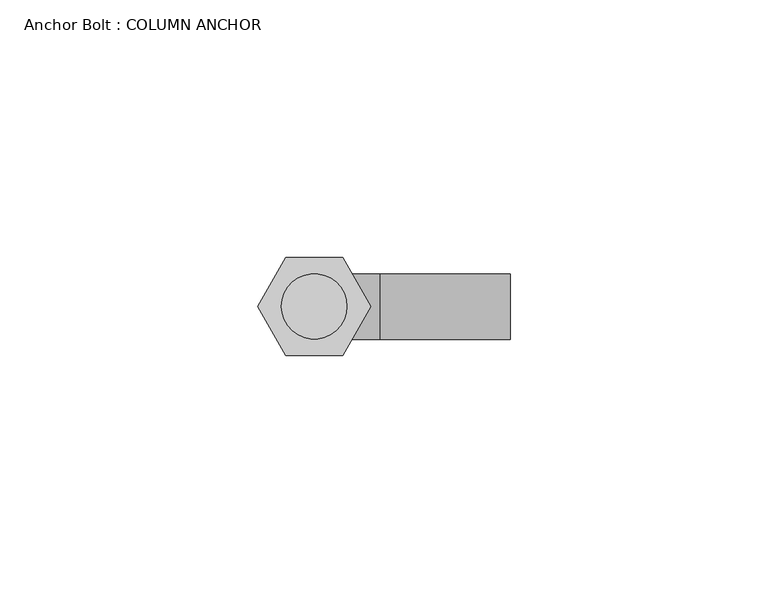
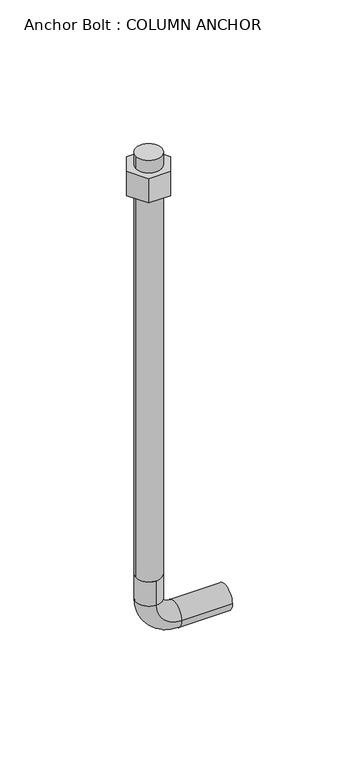
"""IFC4 building model written with IfcOpenShell, lengths in millimetres: fastener geometry, Anchor Bolt : COLUMN ANCHOR."""

from ifc_helpers import new_model, si_unit, point, frame, origin, origin_with_axes, place, context, project, spatial, polyline, circle_curve, ellipse_curve, trimmed, outline, extrude, source, transform, mapped, element, save
from ifc_brep_helpers import plane_surface, cylinder_surface, revolved_surface, advanced_brep


def anchor_bolt_column_anchor_ee5f3531(model_context):
    return source(origin(), model_context, "Body", "SolidModel", [
        advanced_brep(
        [(0.0, 6.35, -203.2), (0.0, 6.35, -215.9), (0.0, -6.35, -215.9), (0.0, -6.35, -203.2), (-6.35, 0.0, -203.2), (6.35, 0.0, -203.2), (12.7, 6.35, -228.6), (12.7, -6.35, -228.6), (38.1, 6.35, -228.6), (38.1, -6.35, -228.6), (-6.35, 0.0, 19.05), (6.35, 0.0, 19.05)],
        [
            (0, 1),
            (1, 2, circle_curve(frame((0.0, 0.0, -215.9), z_axis=(0.0, 0.0, 1.0), x_axis=(0.0, -1.0, 0.0)), 6.35)),
            (2, 3),
            (3, 4, circle_curve(frame((0.0, 0.0, -203.2), z_axis=(0.0, 0.0, -1.0), x_axis=(0.0, -1.0, 0.0)), 6.35)),
            (4, 0, circle_curve(frame((0.0, 0.0, -203.2), z_axis=(0.0, 0.0, -1.0), x_axis=(0.0, -1.0, 0.0)), 6.35)),
            (0, 5, circle_curve(frame((0.0, 0.0, -203.2), z_axis=(0.0, 0.0, -1.0), x_axis=(0.0, -1.0, 0.0)), 6.35)),
            (5, 3, circle_curve(frame((0.0, 0.0, -203.2), z_axis=(0.0, 0.0, -1.0), x_axis=(0.0, -1.0, 0.0)), 6.35)),
            (2, 1, circle_curve(frame((0.0, 0.0, -215.9), z_axis=(0.0, 0.0, 1.0), x_axis=(0.0, -1.0, 0.0)), 6.35)),
            (1, 6, circle_curve(frame((12.7, 6.35, -215.9), z_axis=(0.0, -1.0, 0.0), x_axis=(-1.0, 0.0, 0.0)), 12.7)),
            (6, 7, circle_curve(frame((12.7, 0.0, -228.6), z_axis=(-1.0, 0.0, 0.0), x_axis=(0.0, -1.0, 0.0)), 6.35)),
            (7, 2, circle_curve(frame((12.7, -6.35, -215.9), z_axis=(0.0, 1.0, 0.0), x_axis=(-1.0, 0.0, 0.0)), 12.7)),
            (7, 6, circle_curve(frame((12.7, 0.0, -228.6), z_axis=(-1.0, 0.0, 0.0), x_axis=(0.0, -1.0, 0.0)), 6.35)),
            (8, 9, circle_curve(frame((38.1, 0.0, -228.6), z_axis=(1.0, 0.0, 0.0), x_axis=(0.0, -1.0, 0.0)), 6.35)),
            (9, 8, circle_curve(frame((38.1, 0.0, -228.6), z_axis=(1.0, 0.0, 0.0), x_axis=(0.0, -1.0, 0.0)), 6.35)),
            (6, 8),
            (9, 7),
            (10, 11, circle_curve(frame((0.0, 0.0, 19.05), z_axis=(0.0, 0.0, 1.0), x_axis=(1.0, 0.0, 0.0)), 6.35)),
            (11, 10, circle_curve(frame((0.0, 0.0, 19.05), z_axis=(0.0, 0.0, 1.0), x_axis=(1.0, 0.0, 0.0)), 6.35)),
            (10, 4),
            (5, 11),
        ],
        [
            cylinder_surface(frame((0.0, 0.0, -203.2), z_axis=(0.0, 0.0, 1.0), x_axis=(0.0, -1.0, 0.0)), 6.35),
            revolved_surface(trimmed(ellipse_curve(frame((0.0, 0.0, -215.9), z_axis=(0.0, 0.0, 1.0), x_axis=(0.0, -1.0, 0.0)), 6.35, 6.35), [point((0.0, 6.35, -215.9))], [point((0.0, -6.35, -215.9))], True, "CARTESIAN"), (12.7, 0.0, -215.9), (0.0, -1.0, 0.0)),
            revolved_surface(trimmed(ellipse_curve(frame((0.0, 0.0, -215.9), z_axis=(0.0, 0.0, 1.0), x_axis=(0.0, -1.0, 0.0)), 6.35, 6.35), [point((0.0, -6.35, -215.9))], [point((0.0, 6.35, -215.9))], True, "CARTESIAN"), (12.7, 0.0, -215.9), (0.0, -1.0, 0.0)),
            plane_surface(frame((38.1, 0.0, -228.6), z_axis=(1.0, 0.0, 0.0), x_axis=(0.0, -1.0, 0.0))),
            cylinder_surface(frame((12.7, 0.0, -228.6), z_axis=(-1.0, 0.0, 0.0), x_axis=(0.0, -1.0, 0.0)), 6.35),
            plane_surface(frame((6.35, 0.0, 19.05), z_axis=(0.0, 0.0, 1.0), x_axis=(0.0, 1.0, 0.0))),
            cylinder_surface(frame((0.0, 0.0, -203.2), z_axis=(0.0, 0.0, 1.0), x_axis=(1.0, 0.0, 0.0)), 6.35),
        ],
        [
            (0, [[1, 2, 3, 4, 5]]),
            (0, [[-1, 6, 7, -3, 8]]),
            (1, [[-2, 9, 10, 11]]),
            (2, [[-8, -11, 12, -9]]),
            (3, [[13, 14]]),
            (4, [[-10, 15, -14, 16]]),
            (4, [[-12, -16, -13, -15]]),
            (5, [[17, 18]]),
            (6, [[-17, 19, -4, -7, 20]]),
            (6, [[-18, -20, -6, -5, -19]]),
        ],
    ),
        extrude(outline(polyline([(-10.9985226, 0.0), (-5.4992613, 9.525), (5.4992613, 9.525), (10.9985226, 0.0), (5.4992613, -9.525), (-5.4992613, -9.525), (-10.9985226, 0.0)])), origin_with_axes(), (0.0, 0.0, 1.0), 12.7),
    ])


if __name__ == "__main__":
    model = new_model("IFC4")
    model_context = context("Model", 3, world=origin())
    ifc_project = project(units=[si_unit("LENGTHUNIT", "METRE", prefix="MILLI")], contexts=[model_context])
    site = spatial("IfcSite", under=ifc_project)
    building = spatial("IfcBuilding", under=site)
    placement = place(None, origin())
    anchor_bolt_column_anchor_shape = anchor_bolt_column_anchor_ee5f3531(model_context)
    element("IfcFastener", 1, ObjectType="Anchor Bolt : COLUMN ANCHOR", at=placement, inside=building, context=model_context, shape_type="MappedRepresentation", body=[
        mapped(anchor_bolt_column_anchor_shape, transform((0.0, 0.0, 0.0), x_axis=(1.0, 0.0, 0.0), y_axis=(0.0, 1.0, 0.0), z_axis=(0.0, 0.0, 1.0))),
    ])
    save(model, "model.ifc")

# Revit data of these elements
# Type "Anchor Bolt : COLUMN ANCHOR"
#   Side = 0' - 0 111/256"
#   Radius = 0' - 0 1/4"
#   Length = 0' - 8"
#   Head Size = 0' - 0 3/4"
#   Head Radius = 0' - 0 3/8"
#   Head Height = 0' - 0 1/2"
#   Diameter = 0' - 0 1/2"
#   Default Elevation = 4' - 0"
#   Bolt Material (Size) = 1/2" HOOKED ANCHOR BOLT (8" MIN. EMBED)
# Element 1 (IfcFastener, "Anchor Bolt : COLUMN ANCHOR")
#   Materials on its faces: "1/2\" HOOKED ANCHOR BOLT (8\" MIN. EMBED)"
# Materials
#   "1/2\" HOOKED ANCHOR BOLT (8\" MIN. EMBED)": class "Generic", colour RGB 120 120 120, transparency 0, Cost = 0
